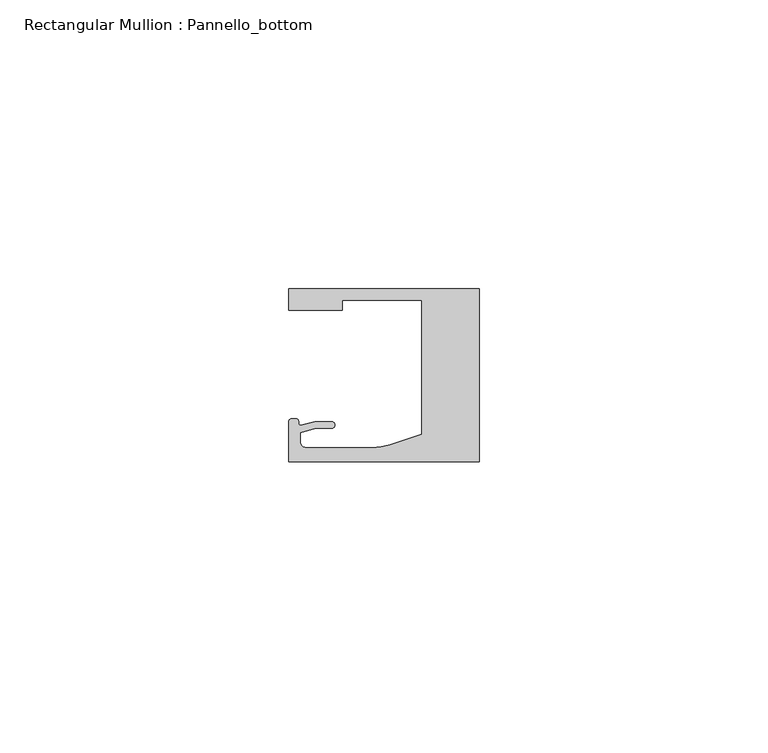
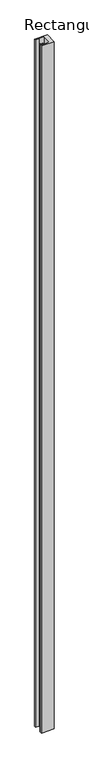
"""IFC4 building model written with IfcOpenShell, lengths in millimetres: member geometry, Rectangular Mullion : Pannello_bottom."""

from ifc_helpers import new_model, si_unit, frame, origin, place, context, project, spatial, polyline, circle_curve, source, transform, mapped, element, save
from ifc_brep_helpers import plane_surface, cylinder_surface, revolved_surface, extruded_surface, spline_curve, advanced_brep


def rectangular_mullion_pannello_bottom_e45f00fa(model_context):
    return source(origin(), model_context, "Body", "AdvancedBrep", [
        advanced_brep(
        [(-33.0, 15.0, 0.0), (-33.0, 11.3000004, 0.0), (-23.700041, 11.3000004, 0.0), (-23.700041, 13.0000004, 0.0), (-9.9999723, 13.0000004, 0.0), (-9.9999723, -10.2367227, 0.0), (-15.4591336, -12.0105099, 0.0), (-18.5493024, -12.4999438, 0.0), (-30.0000002, -12.4999419, 0.0), (-31.0, -11.4999419, 0.0), (-31.0, -9.9121746, 0.0), (-28.3419477, -9.1999523, 0.0), (-25.59998, -9.1999523, 0.0), (-25.59998, -7.9999523, 0.0), (-28.4999305, -7.9999523, 0.0), (-30.9223017, -8.6490241, 0.0), (-33.0000135, -8.0000472, 0.0), (-33.0000135, -15.0, 0.0), (0.0, -15.0, 0.0), (0.0, 15.0, 0.0), (-33.0, 15.0, -1883.9999729), (0.0, 15.0, -1883.9999729), (0.0, -15.0, -1883.9999729), (-33.0000135, -15.0, -1883.9999729), (-33.0000135, -8.0000472, -1883.9999729), (-30.9223017, -8.6490241, -1883.9999729), (-28.4999305, -7.9999523, -1883.9999729), (-25.59998, -7.9999523, -1883.9999729), (-25.59998, -9.1999523, -1883.9999729), (-28.3419477, -9.1999523, -1883.9999729), (-31.0, -9.9121746, -1883.9999729), (-31.0, -11.4999419, -1883.9999729), (-30.0000002, -12.4999419, -1883.9999729), (-18.5493024, -12.4999438, -1883.9999729), (-15.4591336, -12.0105099, -1883.9999729), (-9.9999723, -10.2367227, -1883.9999729), (-9.9999723, 13.0000004, -1883.9999729), (-23.700041, 13.0000004, -1883.9999729), (-23.700041, 11.3000004, -1883.9999729), (-33.0, 11.3000004, -1883.9999729)],
        [
            (0, 1),
            (1, 2),
            (2, 3),
            (3, 4),
            (4, 5),
            (5, 6),
            (6, 7, circle_curve(frame((-18.5493007, -2.4999438, 0.0), z_axis=(0.0, 0.0, -1.0), x_axis=(0.0, -1.0, 0.0)), 10.0)),
            (7, 8),
            (8, 9, circle_curve(frame((-30.0, -11.4999419, 0.0), z_axis=(0.0, 0.0, -1.0), x_axis=(0.0, -1.0, 0.0)), 1.0)),
            (9, 10),
            (10, 11),
            (11, 12),
            (12, 13, circle_curve(frame((-25.59998, -8.5999523, 0.0), z_axis=(0.0, 0.0, 1.0), x_axis=(0.0, -1.0, 0.0)), 0.6)),
            (13, 14),
            (14, 15),
            (15, 16, spline_curve(3, [(-30.9223017, -8.6490241, 0.0), (-31.312054066, -8.717747958, 0.0), (-31.298563602, -8.366228555, 0.0), (-31.305645054, -7.690065204, 0.0), (-31.357433266, -7.563996614, 0.0), (-32.262327879, -7.456527435, 0.0), (-33.0000135, -7.457047519, 0.0), (-33.0000135, -8.0000472, 0.0)], [4, 2, 2, 4], [0.0, 0.001840817752199412, 0.004996616814974408, 0.007702013405570312])),
            (16, 17),
            (17, 18),
            (18, 19),
            (19, 0),
            (20, 21),
            (21, 22),
            (22, 23),
            (23, 24),
            (24, 25, spline_curve(3, [(-33.0000135, -8.0000472, -1883.9999729), (-33.0000135, -7.457047519, -1883.9999729), (-32.262327879, -7.456527435, -1883.9999729), (-31.357433266, -7.563996614, -1883.9999729), (-31.305645054, -7.690065204, -1883.9999729), (-31.298563602, -8.366228555, -1883.9999729), (-31.312054066, -8.717747958, -1883.9999729), (-30.9223017, -8.6490241, -1883.9999729)], [4, 2, 2, 4], [0.0, 0.0027053965905959043, 0.0058611956533709, 0.007702013405570312])),
            (25, 26),
            (26, 27),
            (27, 28, circle_curve(frame((-25.59998, -8.5999523, -1883.9999729), z_axis=(0.0, 0.0, -1.0), x_axis=(0.0, -1.0, 0.0)), 0.6)),
            (28, 29),
            (29, 30),
            (30, 31),
            (31, 32, circle_curve(frame((-30.0, -11.4999419, -1883.9999729), z_axis=(0.0, 0.0, 1.0), x_axis=(0.0, -1.0, 0.0)), 1.0)),
            (32, 33),
            (33, 34, circle_curve(frame((-18.5493007, -2.4999438, -1883.9999729), z_axis=(0.0, 0.0, 1.0), x_axis=(0.0, -1.0, 0.0)), 10.0)),
            (34, 35),
            (35, 36),
            (36, 37),
            (37, 38),
            (38, 39),
            (39, 20),
            (0, 20),
            (39, 1),
            (38, 2),
            (37, 3),
            (36, 4),
            (35, 5),
            (34, 6),
            (33, 7),
            (32, 8),
            (31, 9),
            (30, 10),
            (29, 11),
            (28, 12),
            (27, 13),
            (26, 14),
            (25, 15),
            (24, 16),
            (23, 17),
            (22, 18),
            (21, 19),
        ],
        [
            plane_surface(frame((0.0, -36.2491502, 0.0), z_axis=(0.0, 0.0, 1.0), x_axis=(-1.0, 0.0, 0.0))),
            plane_surface(frame((0.0, -36.2491502, -1883.9999729), z_axis=(0.0, 0.0, -1.0), x_axis=(-1.0, 0.0, 0.0))),
            plane_surface(frame((-33.0, 15.0, 0.0), z_axis=(-1.0, 0.0, 0.0), x_axis=(0.0, 0.0, -1.0))),
            plane_surface(frame((-33.0, 11.3000004, 0.0), z_axis=(0.0, -1.0, 0.0), x_axis=(0.0, 0.0, -1.0))),
            plane_surface(frame((-23.700041, 11.3000004, 0.0), z_axis=(1.0, 0.0, 0.0), x_axis=(0.0, 0.0, -1.0))),
            plane_surface(frame((-23.700041, 13.0000004, 0.0), z_axis=(0.0, -1.0, 0.0), x_axis=(0.0, 0.0, -1.0))),
            plane_surface(frame((-9.9999723, 13.0000004, 0.0), z_axis=(-1.0, 0.0, 0.0), x_axis=(0.0, 0.0, -1.0))),
            plane_surface(frame((-9.9999723, -10.2367227, 0.0), z_axis=(-0.30901670911956314, 0.9510566089801992, 0.0), x_axis=(0.0, 0.0, -1.0))),
            revolved_surface(polyline([(-18.5493007, -12.4999438, -1883.9999729), (-18.5493007, -12.4999438, 0.0)]), (-18.5493007, -2.4999438, 0.0), (0.0, 0.0, -1.0)),
            plane_surface(frame((-18.5493024, -12.4999438, 0.0), z_axis=(1.6923026533778639e-07, 0.9999999999999858, 0.0), x_axis=(0.0, 0.0, -1.0))),
            revolved_surface(polyline([(-30.0, -12.4999419, -1883.9999729), (-30.0, -12.4999419, 0.0)]), (-30.0, -11.4999419, 0.0), (0.0, 0.0, -1.0)),
            plane_surface(frame((-31.0, -11.4999419, 0.0), z_axis=(1.0, 0.0, 0.0), x_axis=(0.0, 0.0, -1.0))),
            plane_surface(frame((-31.0, -9.9121746, 0.0), z_axis=(0.25881883204288636, -0.9659258833782002, 0.0), x_axis=(0.0, 0.0, -1.0))),
            plane_surface(frame((-28.3419477, -9.1999523, 0.0), z_axis=(0.0, -1.0, 0.0), x_axis=(0.0, 0.0, -1.0))),
            cylinder_surface(frame((-25.59998, -8.5999523, 0.0), z_axis=(0.0, 0.0, 1.0), x_axis=(0.0, -1.0, 0.0)), 0.6),
            plane_surface(frame((-25.59998, -7.9999523, 0.0), z_axis=(0.0, 1.0, 0.0), x_axis=(0.0, 0.0, -1.0))),
            plane_surface(frame((-28.4999305, -7.9999523, 0.0), z_axis=(-0.25881883200192934, 0.9659258833891746, 0.0), x_axis=(0.0, 0.0, -1.0))),
            extruded_surface(spline_curve(3, [(-30.9223017, -8.6490241, -1883.9999729), (-31.312054066, -8.717747958, -1883.9999729), (-31.298563602, -8.366228555, -1883.9999729), (-31.305645054, -7.690065204, -1883.9999729), (-31.357433266, -7.563996614, -1883.9999729), (-32.262327879, -7.456527435, -1883.9999729), (-33.0000135, -7.457047519, -1883.9999729), (-33.0000135, -8.0000472, -1883.9999729)], [4, 2, 2, 4], [0.0, 0.001840817752199412, 0.004996616814974408, 0.007702013405570312]), (0.0, 0.0, 1883.9999729), 1883.9999729),
            plane_surface(frame((-33.0000135, -8.0000472, 0.0), z_axis=(-1.0, 0.0, 0.0), x_axis=(0.0, 0.0, -1.0))),
            plane_surface(frame((-33.0000135, -15.0, 0.0), z_axis=(0.0, -1.0, 0.0), x_axis=(0.0, 0.0, -1.0))),
            plane_surface(frame((0.0, -15.0, 0.0), z_axis=(1.0, 0.0, 0.0), x_axis=(0.0, 0.0, -1.0))),
            plane_surface(frame((0.0, 15.0, 0.0), z_axis=(0.0, 1.0, 0.0), x_axis=(0.0, 0.0, -1.0))),
        ],
        [
            (0, [[1, 2, 3, 4, 5, 6, 7, 8, 9, 10, 11, 12, 13, 14, 15, 16, 17, 18, 19, 20]]),
            (1, [[21, 22, 23, 24, 25, 26, 27, 28, 29, 30, 31, 32, 33, 34, 35, 36, 37, 38, 39, 40]]),
            (2, [[-1, 41, -40, 42]]),
            (3, [[-2, -42, -39, 43]]),
            (4, [[-3, -43, -38, 44]]),
            (5, [[-4, -44, -37, 45]]),
            (6, [[-5, -45, -36, 46]]),
            (7, [[-6, -46, -35, 47]]),
            (8, [[-7, -47, -34, 48]]),
            (9, [[-8, -48, -33, 49]]),
            (10, [[-9, -49, -32, 50]]),
            (11, [[-10, -50, -31, 51]]),
            (12, [[-11, -51, -30, 52]]),
            (13, [[-12, -52, -29, 53]]),
            (14, [[-13, -53, -28, 54]]),
            (15, [[-14, -54, -27, 55]]),
            (16, [[-15, -55, -26, 56]]),
            (17, [[-16, -56, -25, 57]]),
            (18, [[-17, -57, -24, 58]]),
            (19, [[-18, -58, -23, 59]]),
            (20, [[-19, -59, -22, 60]]),
            (21, [[-20, -60, -21, -41]]),
        ],
    ),
    ])


if __name__ == "__main__":
    model = new_model("IFC4")
    model_context = context("Model", 3, world=origin())
    ifc_project = project(units=[si_unit("LENGTHUNIT", "METRE", prefix="MILLI")], contexts=[model_context])
    site = spatial("IfcSite", under=ifc_project)
    building = spatial("IfcBuilding", under=site)
    placement = place(None, origin())
    rectangular_mullion_pannello_bottom_shape = rectangular_mullion_pannello_bottom_e45f00fa(model_context)
    element("IfcMember", 1, ObjectType="Rectangular Mullion : Pannello_bottom", at=placement, inside=building, context=model_context, shape_type="MappedRepresentation", body=[
        mapped(rectangular_mullion_pannello_bottom_shape, transform((0.0, 0.0, 0.0), x_axis=(1.0, 0.0, 0.0), y_axis=(0.0, 1.0, 0.0), z_axis=(0.0, 0.0, 1.0))),
    ])
    save(model, "model.ifc")

# Revit data of these elements
# Type "Rectangular Mullion : Pannello_bottom"
#   built-in parameter 1007322 = 0.0984252 (stored number, unit not read)
#   built-in parameter 1007321 = 0.0328083 (stored number, unit not read)
#   built-in parameter 1007320 = 0 (stored number, unit not read)
